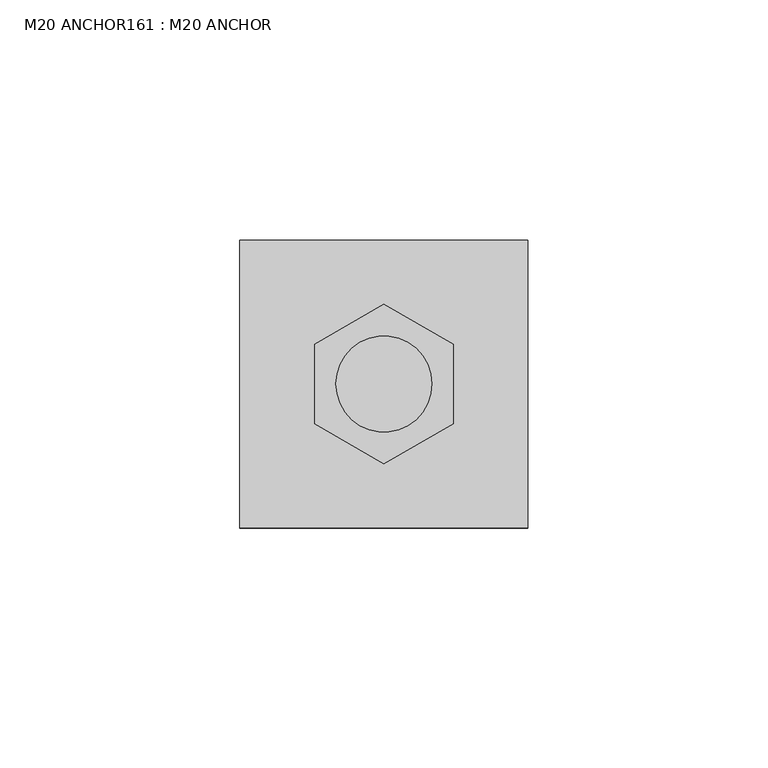
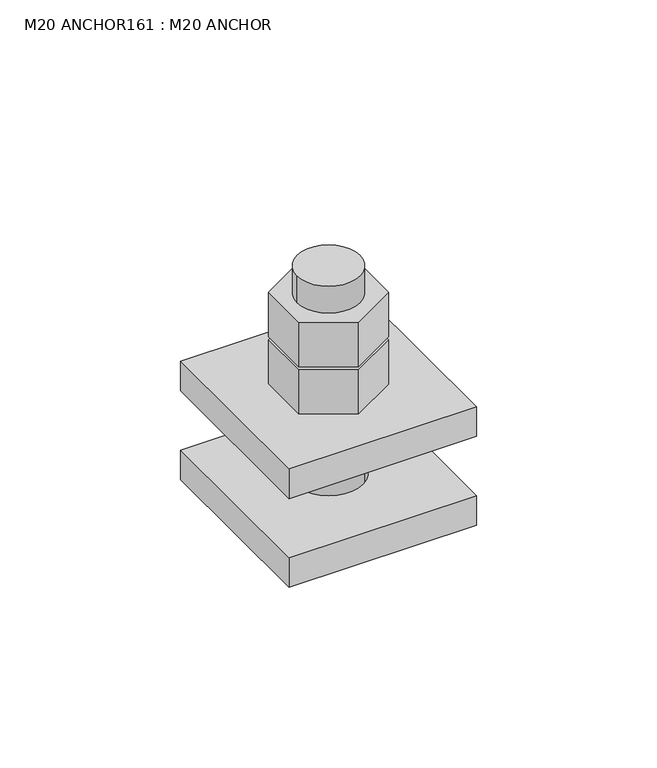
"""IFC4 building model written with IfcOpenShell, lengths in millimetres: fastener geometry, M20 ANCHOR161 : M20 ANCHOR."""

import ifcopenshell
import ifcopenshell.guid

model = None  # the IFC model being written
_history = None  # IfcOwnerHistory: only IFC2X3 demands one
_inside = {}  # id of a spatial element -> (the spatial element, [elements in it])
_under = {}  # id of a project, library or spatial element -> (it, [spatial elements below it])
_declared = {}  # id of a project -> (the project, [libraries it declares])
_typed = {}  # id of a type object -> (the type object, [elements of that type])
_made_of = {}  # id of a material, layer set ... -> (it, [elements and type objects made of it])


def new_model(schema):
    """Start an empty IFC model of exactly this schema.

    Asked for "IFC4X3", IfcOpenShell would pick the latest addendum, in which some entities
    have other attributes; the version numbers below select the first issue.
    IFC2X3 requires an IfcOwnerHistory on every rooted entity: one is made here for all.
    """
    global model, _history
    if schema == "IFC4X3":
        model = ifcopenshell.file(schema_version=(4, 3, 0, 0))
    else:
        model = ifcopenshell.file(schema=schema)
    _inside.clear()
    _under.clear()
    _declared.clear()
    _typed.clear()
    _made_of.clear()
    _history = None
    if model.schema == "IFC2X3":
        org = make("IfcOrganization", Name="unknown")
        user = make(
            "IfcPersonAndOrganization",
            ThePerson=make("IfcPerson", FamilyName="unknown"),
            TheOrganization=org,
        )
        app = make(
            "IfcApplication",
            ApplicationDeveloper=org,
            Version="unknown",
            ApplicationFullName="unknown",
            ApplicationIdentifier="unknown",
        )
        _history = make(
            "IfcOwnerHistory",
            OwningUser=user,
            OwningApplication=app,
            ChangeAction="ADDED",
            CreationDate=0,
        )
    return model


def make(cls, **values):
    """One entity of the class cls with the attributes given. An attribute that is None is left unset."""
    return model.create_entity(
        cls, **{name: value for name, value in values.items() if value is not None}
    )


def rooted(cls, **values):
    """An entity with a GlobalId (a new one), such as an element, a storey or a relation."""
    return make(cls, GlobalId=ifcopenshell.guid.new(), OwnerHistory=_history, **values)


def si_unit(unit_type, name, prefix=None):
    """IfcSIUnit, for example si_unit("LENGTHUNIT", "METRE", prefix="MILLI")."""
    return make("IfcSIUnit", UnitType=unit_type, Prefix=prefix, Name=name)


def assignment(units):
    """IfcUnitAssignment: the units of a project."""
    return None if units is None else make("IfcUnitAssignment", Units=units)


def point(xyz):
    """IfcCartesianPoint."""
    return None if xyz is None else make("IfcCartesianPoint", Coordinates=xyz)


def direction(xyz):
    """IfcDirection."""
    return None if xyz is None else make("IfcDirection", DirectionRatios=xyz)


def frame(location, z_axis=None, x_axis=None):
    """IfcAxis2Placement3D, a coordinate frame: its origin and axes. An axis left out is left unset."""
    return make(
        "IfcAxis2Placement3D",
        Location=point(location),
        Axis=direction(z_axis),
        RefDirection=direction(x_axis),
    )


def frame_2d(location, x_axis=None):
    """IfcAxis2Placement2D, a coordinate frame in the plane: its origin and x axis."""
    return make(
        "IfcAxis2Placement2D", Location=point(location), RefDirection=direction(x_axis)
    )


def origin():
    """The frame at (0, 0, 0) with its axes left unset."""
    return frame((0.0, 0.0, 0.0))


def place(relative_to, where):
    """IfcLocalPlacement: puts the frame where relative to a parent placement (None: the world)."""
    return make(
        "IfcLocalPlacement", PlacementRelTo=relative_to, RelativePlacement=where
    )


def context(
    kind, dimensions, precision=None, world=None, true_north=None, identifier=None
):
    """IfcGeometricRepresentationContext, for example the 3D "Model" context."""
    return make(
        "IfcGeometricRepresentationContext",
        ContextIdentifier=identifier,
        ContextType=kind,
        CoordinateSpaceDimension=dimensions,
        Precision=precision,
        WorldCoordinateSystem=world,
        TrueNorth=true_north,
    )


def project(units=None, contexts=None):
    """IfcProject with its units and contexts."""
    return rooted(
        "IfcProject",
        Name="project",
        RepresentationContexts=contexts,
        UnitsInContext=assignment(units),
    )


def spatial(cls, under=None, at=None, **own):
    """A site, building, storey or space (cls), placed at a placement, below another one or the project."""
    s = rooted(cls, ObjectPlacement=at, **own)
    if under is not None:
        _under.setdefault(under.id(), (under, []))[1].append(s)
    return s


def polyline(points):
    """IfcPolyline through the points."""
    return make("IfcPolyline", Points=[point(p) for p in points])


def circle_curve(where, radius):
    """IfcCircle in the frame where."""
    return make("IfcCircle", Position=where, Radius=radius)


def trimmed(basis, trim1, trim2, sense, master):
    """IfcTrimmedCurve: the piece of a basis curve between two trims."""
    return make(
        "IfcTrimmedCurve",
        BasisCurve=basis,
        Trim1=trim1,
        Trim2=trim2,
        SenseAgreement=sense,
        MasterRepresentation=master,
    )


def segment(curve, same_sense, transition):
    """IfcCompositeCurveSegment."""
    return make(
        "IfcCompositeCurveSegment",
        Transition=transition,
        SameSense=same_sense,
        ParentCurve=curve,
    )


def composite_curve(segments, self_intersect=None):
    """IfcCompositeCurve: segments joined end to end."""
    return make("IfcCompositeCurve", Segments=segments, SelfIntersect=self_intersect)


def outline(outer, holes=None, kind="AREA"):
    """IfcArbitraryClosedProfileDef: a profile drawn as a closed curve; with holes, ...WithVoids."""
    if holes is None:
        return make("IfcArbitraryClosedProfileDef", ProfileType=kind, OuterCurve=outer)
    return make(
        "IfcArbitraryProfileDefWithVoids",
        ProfileType=kind,
        OuterCurve=outer,
        InnerCurves=holes,
    )


def extrude(swept, where, along, depth):
    """IfcExtrudedAreaSolid: the profile swept, set in the frame where, extruded along a direction by depth."""
    return make(
        "IfcExtrudedAreaSolid",
        SweptArea=swept,
        Position=where,
        ExtrudedDirection=direction(along),
        Depth=depth,
    )


def shape(context_of_items, identifier, shape_type, items):
    """IfcShapeRepresentation: the items that make up one representation, for example the "Body"."""
    return make(
        "IfcShapeRepresentation",
        ContextOfItems=context_of_items,
        RepresentationIdentifier=identifier,
        RepresentationType=shape_type,
        Items=items,
    )


def source(mapping_origin, context_of_items, identifier, shape_type, items):
    """IfcRepresentationMap: a shape defined once, which mapped items show again and again."""
    return make(
        "IfcRepresentationMap",
        MappingOrigin=mapping_origin,
        MappedRepresentation=shape(context_of_items, identifier, shape_type, items),
    )


def transform(
    local_origin,
    x_axis=None,
    y_axis=None,
    z_axis=None,
    scale=None,
    scale2=None,
    scale3=None,
    uniform=True,
):
    """IfcCartesianTransformationOperator3D, or its non-uniform kind. x_axis, y_axis, z_axis: its Axis1, 2, 3."""
    if uniform:
        return make(
            "IfcCartesianTransformationOperator3D",
            Axis1=direction(x_axis),
            Axis2=direction(y_axis),
            LocalOrigin=point(local_origin),
            Scale=scale,
            Axis3=direction(z_axis),
        )
    return make(
        "IfcCartesianTransformationOperator3DnonUniform",
        Axis1=direction(x_axis),
        Axis2=direction(y_axis),
        LocalOrigin=point(local_origin),
        Scale=scale,
        Axis3=direction(z_axis),
        Scale2=scale2,
        Scale3=scale3,
    )


def mapped(mapping_source, mapping_target):
    """IfcMappedItem: shows the shape of a source again, moved by a transform."""
    return make(
        "IfcMappedItem", MappingSource=mapping_source, MappingTarget=mapping_target
    )


def made_of(thing, what):
    """Note that an element or type object is made of a material, layer set ...; save() writes the relation."""
    if what is not None:
        _made_of.setdefault(what.id(), (what, []))[1].append(thing)
    return thing


def element(
    cls,
    number,
    at=None,
    inside=None,
    cuts=None,
    type_object=None,
    material=None,
    context=None,
    identifier="Body",
    shape_type=None,
    held_by="IfcProductDefinitionShape",
    body=None,
    shapes=None,
    **own,
):
    """One element of the class cls, such as IfcWall. Its Tag is "e" and its number.

    at: its placement. inside: the storey or other place that contains it. cuts: it is an
    opening in that element (IfcRelVoidsElement). A single representation is given by context,
    identifier, shape_type and body (its items); several are given by shapes. held_by: the class
    of the entity that holds the representations. save() writes the other relations.
    """
    e = rooted(cls, Tag="e%d" % number, ObjectPlacement=at, **own)
    if body is not None:
        shapes = [shape(context, identifier, shape_type, body)]
    if shapes is not None:
        e.Representation = make(held_by, Representations=shapes)
    if inside is not None:
        _inside.setdefault(inside.id(), (inside, []))[1].append(e)
    if cuts is not None:
        rooted(
            "IfcRelVoidsElement", RelatingBuildingElement=cuts, RelatedOpeningElement=e
        )
    if type_object is not None:
        _typed.setdefault(type_object.id(), (type_object, []))[1].append(e)
    return made_of(e, material)


def aggregate(whole, parts):
    """IfcRelAggregates: a whole, such as a stair, and the parts it consists of."""
    return rooted("IfcRelAggregates", RelatingObject=whole, RelatedObjects=parts)


def save(model, path):
    """Write the relations noted so far, then the file.

    IfcRelAggregates (storeys below a building ...), IfcRelContainedInSpatialStructure (elements
    in a storey), IfcRelDefinesByType, IfcRelAssociatesMaterial and IfcRelDeclares: one each for
    every whole, place, type object, material and project.
    """
    for whole, parts in _under.values():
        aggregate(whole, parts)
    for where, things in _inside.values():
        rooted(
            "IfcRelContainedInSpatialStructure",
            RelatedElements=things,
            RelatingStructure=where,
        )
    for kind, things in _typed.values():
        rooted("IfcRelDefinesByType", RelatedObjects=things, RelatingType=kind)
    for what, things in _made_of.values():
        rooted("IfcRelAssociatesMaterial", RelatedObjects=things, RelatingMaterial=what)
    for by, libraries in _declared.values():
        rooted("IfcRelDeclares", RelatingContext=by, RelatedDefinitions=libraries)
    model.write(path)


def m20_anchor161_m20_anchor_832bce39(model_context):
    return source(origin(), model_context, "Body", "SweptSolid", [
        extrude(outline(polyline([(6008.0855968, 19453.9464399), (6008.0855968, 19470.5835027), (6022.4937158, 19478.9020341), (6036.9018348, 19470.5835027), (6036.9018348, 19453.9464399), (6022.4937158, 19445.6279085), (6008.0855968, 19453.9464399)]), holes=[composite_curve([segment(trimmed(circle_curve(frame_2d((6022.4937158, 19462.2649713)), 10.0), [point((6032.4937158, 19462.2649713))], [point((6012.4937158, 19462.2649713))], True, "CARTESIAN"), True, "CONTINUOUS"), segment(trimmed(circle_curve(frame_2d((6022.4937158, 19462.2649713)), 10.0), [point((6012.4937158, 19462.2649713))], [point((6032.4937158, 19462.2649713))], True, "CARTESIAN"), True, "CONTINUOUS")], self_intersect=False)]), frame((0.0, 0.0, 246.0), z_axis=(0.0, 0.0, 1.0), x_axis=(1.0, 0.0, 0.0)), (0.0, 0.0, 1.0), 15.0),
        extrude(outline(polyline([(6008.0855968, 19453.9464399), (6008.0855968, 19470.5835027), (6022.4937158, 19478.9020341), (6036.9018348, 19470.5835027), (6036.9018348, 19453.9464399), (6022.4937158, 19445.6279085), (6008.0855968, 19453.9464399)]), holes=[composite_curve([segment(trimmed(circle_curve(frame_2d((6022.4937158, 19462.2649713)), 10.0), [point((6032.4937158, 19462.2649713))], [point((6012.4937158, 19462.2649713))], True, "CARTESIAN"), True, "CONTINUOUS"), segment(trimmed(circle_curve(frame_2d((6022.4937158, 19462.2649713)), 10.0), [point((6012.4937158, 19462.2649713))], [point((6032.4937158, 19462.2649713))], True, "CARTESIAN"), True, "CONTINUOUS")], self_intersect=False)]), frame((0.0, 0.0, 230.0), z_axis=(0.0, 0.0, 1.0), x_axis=(1.0, 0.0, 0.0)), (0.0, 0.0, 1.0), 15.0),
        extrude(outline(composite_curve([segment(trimmed(circle_curve(frame_2d((6022.4937158, 19462.2649713)), 10.0), [point((6032.4937158, 19462.2649713))], [point((6012.4937158, 19462.2649713))], False, "CARTESIAN"), True, "CONTINUOUS"), segment(trimmed(circle_curve(frame_2d((6022.4937158, 19462.2649713)), 10.0), [point((6012.4937158, 19462.2649713))], [point((6032.4937158, 19462.2649713))], False, "CARTESIAN"), True, "CONTINUOUS")], self_intersect=False)), frame((0.0, 0.0, 190.0), z_axis=(0.0, 0.0, 1.0), x_axis=(1.0, 0.0, 0.0)), (0.0, 0.0, 1.0), 80.0),
        extrude(outline(polyline([(5992.4937158, 19432.2649713), (5992.4937158, 19492.2649713), (6052.4937158, 19492.2649713), (6052.4937158, 19432.2649713), (5992.4937158, 19432.2649713)]), holes=[composite_curve([segment(trimmed(circle_curve(frame_2d((6022.4937158, 19462.2649713)), 11.0), [point((6033.4937158, 19462.2649713))], [point((6011.4937158, 19462.2649713))], True, "CARTESIAN"), True, "CONTINUOUS"), segment(trimmed(circle_curve(frame_2d((6022.4937158, 19462.2649713)), 11.0), [point((6011.4937158, 19462.2649713))], [point((6033.4937158, 19462.2649713))], True, "CARTESIAN"), True, "CONTINUOUS")], self_intersect=False)]), frame((0.0, 0.0, 190.0), z_axis=(0.0, 0.0, 1.0), x_axis=(1.0, 0.0, 0.0)), (0.0, 0.0, 1.0), 10.0),
        extrude(outline(polyline([(5992.4937158, 19432.2649713), (5992.4937158, 19492.2649713), (6052.4937158, 19492.2649713), (6052.4937158, 19432.2649713), (5992.4937158, 19432.2649713)]), holes=[composite_curve([segment(trimmed(circle_curve(frame_2d((6022.4937158, 19462.2649713)), 11.0), [point((6033.4937158, 19462.2649713))], [point((6011.4937158, 19462.2649713))], True, "CARTESIAN"), True, "CONTINUOUS"), segment(trimmed(circle_curve(frame_2d((6022.4937158, 19462.2649713)), 11.0), [point((6011.4937158, 19462.2649713))], [point((6033.4937158, 19462.2649713))], True, "CARTESIAN"), True, "CONTINUOUS")], self_intersect=False)]), frame((0.0, 0.0, 220.0), z_axis=(0.0, 0.0, 1.0), x_axis=(1.0, 0.0, 0.0)), (0.0, 0.0, 1.0), 10.0),
    ])


if __name__ == "__main__":
    model = new_model("IFC4")
    model_context = context("Model", 3, world=origin())
    ifc_project = project(units=[si_unit("LENGTHUNIT", "METRE", prefix="MILLI")], contexts=[model_context])
    site = spatial("IfcSite", under=ifc_project)
    building = spatial("IfcBuilding", under=site)
    placement = place(None, origin())
    m20_anchor161_m20_anchor_shape = m20_anchor161_m20_anchor_832bce39(model_context)
    element("IfcFastener", 1, ObjectType="M20 ANCHOR161 : M20 ANCHOR", at=placement, inside=building, context=model_context, shape_type="MappedRepresentation", body=[
        mapped(m20_anchor161_m20_anchor_shape, transform((0.0, 0.0, 0.0), x_axis=(1.0, 0.0, 0.0), y_axis=(0.0, 1.0, 0.0), z_axis=(0.0, 0.0, 1.0))),
    ])
    save(model, "model.ifc")
